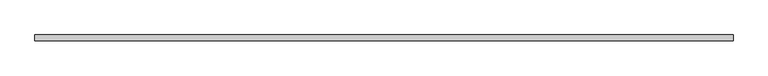
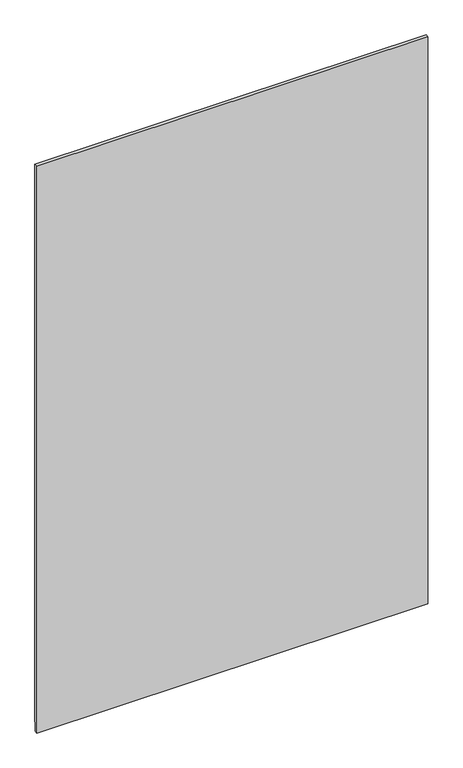
"""IFC4 building model written with IfcOpenShell, lengths in millimetres: proxy geometry, Generic Models 7:Generic Models 1:5:Generic Models 1:5 : Generic Models 7:Generic Models 1:337419:10 : Generic Models 7:Generic Models 1:5:Generic Models 1:5 : Generic Models 7:Generic Models 1:337419:311462."""

from ifc_helpers import new_model, si_unit, frame, origin, place, context, project, spatial, polyline, outline, extrude, source, transform, mapped, element, save


def generic_models_5f0b78a4(model_context):
    return source(origin(), model_context, "Body", "SweptSolid", [
        extrude(outline(polyline([(-579038.7913841, 30.4457208), (-579038.7913841, 3712.5974457), (-579018.7195842, 3712.5974457), (-579018.7195842, 90.8175588), (-579020.7152542, 88.8218888), (-579020.7152542, 30.4457208), (-579038.7913841, 30.4457208)])), frame((593758.7242239, 0.0, 0.0), z_axis=(1.0, 0.0, 0.0), x_axis=(0.0, 1.0, 0.0)), (0.0, 0.0, 1.0), 2403.4750001),
    ])


if __name__ == "__main__":
    model = new_model("IFC4")
    model_context = context("Model", 3, world=origin())
    ifc_project = project(units=[si_unit("LENGTHUNIT", "METRE", prefix="MILLI")], contexts=[model_context])
    site = spatial("IfcSite", under=ifc_project)
    building = spatial("IfcBuilding", under=site)
    placement = place(None, origin())
    generic_models_shape = generic_models_5f0b78a4(model_context)
    element("IfcBuildingElementProxy", 1, Name="Generic Models 7:Generic Models 1:5:Generic Models 1:5 : Generic Models 7:Generic Models 1:337419:10 : Generic Models 7:Generic Models 1:5:Generic Models 1:5 : Generic Models 7:Generic Models 1:337419:311462", ObjectType="Generic Models 7:Generic Models 1:5:Generic Models 1:5 : Generic Models 7:Generic Models 1:337419:10 : Generic Models 7:Generic Models 1:5:Generic Models 1:5 : Generic Models 7:Generic Models 1:337419:311462", at=placement, inside=building, context=model_context, shape_type="MappedRepresentation", body=[
        mapped(generic_models_shape, transform((0.0, 0.0, 0.0), x_axis=(1.0, 0.0, 0.0), y_axis=(0.0, 1.0, 0.0), z_axis=(0.0, 0.0, 1.0))),
    ])
    save(model, "model.ifc")

# Revit data of these elements
# Type "Generic Models 7:Generic Models 1:5:Generic Models 1:5 : Generic Models 7:Generic Models 1:337419:10 : Generic Models 7:Generic Models 1:5:Generic Models 1:5 : Generic Models 7:Generic Models 1:337419:311462"
#   NameOverride = "Generic Models 7:Generic Models 1:5:Generic Models 1:5 : Generic Models 7:Generic Models 1:337419:311462"
#   ObjectTypeOverride = "Generic Models 1:5 : Generic Models 7:Generic Models 1:337419"
#   Reference = "Generic Models 1"
#   Tag = "311462"
# Element 1 (IfcBuildingElementProxy, "Generic Models 7:Generic Models 1:5:Generic Models 1:5 : Generic Models 7:Generic Models 1:337419:10 : Generic Models 7:Generic Models 1:5:Generic Models 1:5 : Generic Models 7:Generic Models 1:337419:311462")
#   Materials on its faces: "1\" MINERAL WOOL BOARD INSULATION - BLACK MAT FACER"
# Materials
#   "1\" MINERAL WOOL BOARD INSULATION - BLACK MAT FACER": class "Unassigned", colour RGB 205 188 106, transparency 0, Cost = 0
